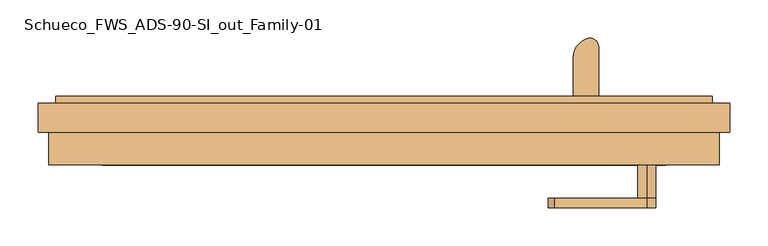
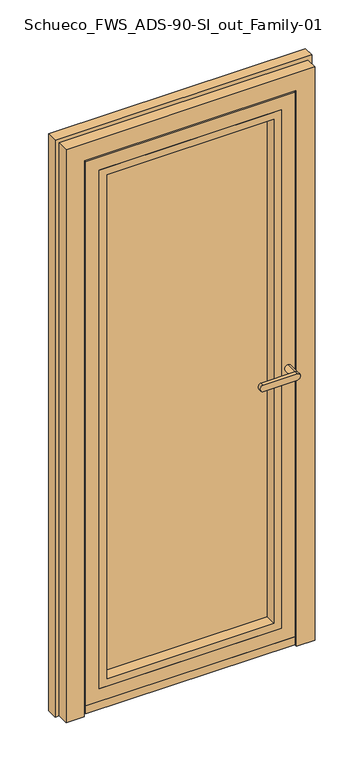
"""IFC4 building model written with IfcOpenShell, lengths in millimetres: door geometry, Schueco_FWS_ADS-90-SI_out_Family-01 : FWS SI insert unit."""

from ifc_helpers import new_model, si_unit, point, frame, frame_2d, origin, place, context, project, spatial, polyline, circle_curve, ellipse_curve, trimmed, segment, composite_curve, outline, extrude, faceted_brep, source, transform, mapped, element, save
from ifc_brep_helpers import plane_surface, cylinder_surface, extruded_surface, advanced_brep


def schueco_fws_ads_90_si_out_family_01_926161e4(model_context):
    return source(origin(), model_context, "Body", "SolidModel", [
        extrude(outline(composite_curve([segment(polyline([(248.3326764, 8.9997177), (248.3326764, 59.1618682)]), True, "CONTINUOUS"), segment(trimmed(circle_curve(frame_2d((275.5110941, 59.1618682)), 27.1784177), [point((248.3326764, 59.1618682))], [point((265.9739985, 84.6120194))], False, "CARTESIAN"), True, "CONTINUOUS"), segment(trimmed(circle_curve(frame_2d((270.0514995, 73.7310321)), 11.6198924), [point((265.9739985, 84.6120194))], [point((281.6713919, 73.7310321))], False, "CARTESIAN"), True, "CONTINUOUS"), segment(polyline([(281.6713919, 73.7310321), (281.6713919, 8.9997177), (248.3326764, 8.9997177)]), True, "CONTINUOUS")], self_intersect=False)), frame((0.0, 0.0, 2043.9340013), z_axis=(0.0, 0.0, 1.0), x_axis=(1.0, 0.0, 0.0)), (0.0, 0.0, 1.0), 4.0),
        extrude(outline(polyline([(248.3326764, 12.9997177), (281.6713919, 12.9997177), (281.6713919, 8.9997177), (248.3326764, 8.9997177), (248.3326764, 12.9997177)])), frame((0.0, 0.0, 2013.9340013), z_axis=(0.0, 0.0, 1.0), x_axis=(1.0, 0.0, 0.0)), (0.0, 0.0, 1.0), 30.0),
        extrude(outline(polyline([(248.3326764, 12.9997177), (281.6713919, 12.9997177), (281.6713919, 8.9997177), (248.3326764, 8.9997177), (248.3326764, 12.9997177)])), frame((0.0, 0.0, 56.9340013), z_axis=(0.0, 0.0, 1.0), x_axis=(1.0, 0.0, 0.0)), (0.0, 0.0, 1.0), 30.0),
        extrude(outline(composite_curve([segment(polyline([(248.3326764, 8.9997177), (248.3326764, 59.1618682)]), True, "CONTINUOUS"), segment(trimmed(circle_curve(frame_2d((275.5110941, 59.1618682)), 27.1784177), [point((248.3326764, 59.1618682))], [point((265.9739985, 84.6120194))], False, "CARTESIAN"), True, "CONTINUOUS"), segment(trimmed(circle_curve(frame_2d((270.0514995, 73.7310321)), 11.6198924), [point((265.9739985, 84.6120194))], [point((281.6713919, 73.7310321))], False, "CARTESIAN"), True, "CONTINUOUS"), segment(polyline([(281.6713919, 73.7310321), (281.6713919, 8.9997177), (248.3326764, 8.9997177)]), True, "CONTINUOUS")], self_intersect=False)), frame((0.0, 0.0, 52.9340013), z_axis=(0.0, 0.0, 1.0), x_axis=(1.0, 0.0, 0.0)), (0.0, 0.0, 1.0), 4.0),
        advanced_brep(
        [(277.717076, 57.5977179, 2043.9340013), (252.282924, 72.2821425, 2043.9340013), (277.717076, 57.5977179, 56.9340013), (252.282924, 72.2821425, 56.9340013)],
        [
            (0, 1, ellipse_curve(frame((265.0, 64.9399302, 2043.9340013), z_axis=(0.0, 0.0, 1.0000000000000002), x_axis=(0.5000002582658958, 0.866025254674503, 0.0)), 21.5840887, 14.6844171)),
            (1, 0, ellipse_curve(frame((265.0, 64.9399302, 2043.9340013), z_axis=(0.0, 0.0, 1.0000000000000002), x_axis=(0.5000002582658958, 0.866025254674503, 0.0)), 21.5840887, 14.6844171)),
            (2, 3, ellipse_curve(frame((265.0, 64.9399302, 56.9340013), z_axis=(0.0, 0.0, -1.0000000000000002), x_axis=(-0.866025254674503, 0.5000002582658958, 0.0)), 14.6844171, 21.5840887)),
            (3, 2, ellipse_curve(frame((265.0, 64.9399302, 56.9340013), z_axis=(0.0, 0.0, -1.0000000000000002), x_axis=(-0.866025254674503, 0.5000002582658958, 0.0)), 14.6844171, 21.5840887)),
            (0, 2),
            (3, 1),
        ],
        [
            plane_surface(frame((252.282924, 72.2821425, 2043.9340013), z_axis=(0.0, 0.0, 1.0000000000000002), x_axis=(0.5000002582658958, 0.866025254674503, 0.0))),
            plane_surface(frame((252.282924, 72.2821425, 56.9340013), z_axis=(0.0, 0.0, -1.0000000000000002), x_axis=(-0.5000002582658958, -0.866025254674503, 0.0))),
            extruded_surface(trimmed(ellipse_curve(frame((265.0, 64.9399302, 56.9340013), z_axis=(0.0, 0.0, -1.0000000000000002), x_axis=(-0.866025254674503, 0.5000002582658958, 0.0)), 14.6844171, 21.5840887), [point((252.282924, 72.2821425, 56.9340013))], [point((277.717076, 57.5977179, 56.9340013))], True, "CARTESIAN"), (0.0, 0.0, -1987.0), 1987.0),
            extruded_surface(trimmed(ellipse_curve(frame((265.0, 64.9399302, 56.9340013), z_axis=(0.0, 0.0, -1.0000000000000002), x_axis=(-0.866025254674503, 0.5000002582658958, 0.0)), 14.6844171, 21.5840887), [point((277.717076, 57.5977179, 56.9340013))], [point((252.282924, 72.2821425, 56.9340013))], True, "CARTESIAN"), (0.0, 0.0, -1987.0), 1987.0),
        ],
        [
            (0, [[1, 2]]),
            (1, [[3, 4]]),
            (2, [[5, -4, 6, -1]]),
            (3, [[-6, -3, -5, -2]]),
        ],
    ),
        advanced_brep(
        [(345.0, -137.0002518, 1038.0113692), (345.0, -137.0002518, 1061.9886308), (223.3382074, -137.0002518, 1061.9886308), (223.3382074, -137.0002518, 1038.0113692), (345.0, -124.5001648, 1061.9886308), (345.0, -124.5001648, 1038.0113692), (223.3382074, -124.5001648, 1038.0113692), (223.3382074, -124.5001648, 1061.9886308), (345.0, -81.0002823, 1038.0113692), (345.0, -81.0002823, 1061.9886308)],
        [
            (0, 1, circle_curve(frame((345.0, -137.0002518, 1050.0), z_axis=(0.0, -1.0, 0.0), x_axis=(0.0, 0.0, 1.0)), 11.9886308)),
            (1, 2),
            (2, 3, ellipse_curve(frame((223.3382074, -137.0002518, 1050.0), z_axis=(0.0, -1.0, 0.0), x_axis=(0.0, 0.0, -1.0)), 11.9886308, 7.9050795)),
            (3, 0),
            (4, 5, circle_curve(frame((345.0, -124.5001648, 1050.0), z_axis=(0.0, -1.0, 0.0), x_axis=(0.0, 0.0, 1.0)), 11.9886308)),
            (5, 6),
            (6, 7, ellipse_curve(frame((223.3382074, -124.5001648, 1050.0), z_axis=(0.0, 1.0, 0.0), x_axis=(0.0, 0.0, -1.0)), 11.9886308, 7.9050795)),
            (7, 4),
            (3, 6),
            (5, 0),
            (2, 7),
            (1, 4),
            (5, 4, circle_curve(frame((345.0, -124.5001648, 1050.0), z_axis=(0.0, -1.0, 0.0), x_axis=(0.0, 0.0, 1.0)), 11.9886308)),
            (8, 9, circle_curve(frame((345.0, -81.0002823, 1050.0), z_axis=(0.0, 1.0, 0.0), x_axis=(0.0, 0.0, 1.0)), 11.9886308)),
            (9, 8, circle_curve(frame((345.0, -81.0002823, 1050.0), z_axis=(0.0, 1.0, 0.0), x_axis=(0.0, 0.0, 1.0)), 11.9886308)),
            (8, 5),
            (4, 9),
        ],
        [
            plane_surface(frame((223.3382074, -137.0002518, 1038.0113692), z_axis=(0.0, -1.0, 0.0), x_axis=(-1.0, 0.0, 0.0))),
            plane_surface(frame((223.3382074, -124.5001648, 1038.0113692), z_axis=(0.0, 1.0, 0.0), x_axis=(1.0, 0.0, 0.0))),
            plane_surface(frame((345.0, -137.0002518, 1038.0113692), z_axis=(0.0, 0.0, -1.0), x_axis=(0.0, 1.0, 0.0))),
            extruded_surface(trimmed(ellipse_curve(frame((223.3382074, -124.5001648, 1050.0), z_axis=(0.0, 1.0, 0.0), x_axis=(0.0, 0.0, -1.0)), 11.9886308, 7.9050795), [point((223.3382074, -124.5001648, 1038.0113692))], [point((223.3382074, -124.5001648, 1061.9886308))], True, "CARTESIAN"), (0.0, 12.500086999999994, 0.0), 12.500086999999994),
            plane_surface(frame((223.3382074, -137.0002518, 1061.9886308), z_axis=(0.0, 0.0, 1.0), x_axis=(0.0, 1.0, 0.0))),
            cylinder_surface(frame((345.0, -124.5001648, 1050.0), z_axis=(0.0, -1.0, 0.0), x_axis=(0.0, 0.0, 1.0)), 11.9886308),
            plane_surface(frame((345.0, -81.0002823, 1061.9886308), z_axis=(0.0, 1.0, 0.0), x_axis=(-1.0, 0.0, 0.0))),
            cylinder_surface(frame((345.0, -81.0002823, 1050.0), z_axis=(0.0, -1.0, 0.0), x_axis=(0.0, 0.0, 1.0)), 11.9886308),
        ],
        [
            (0, [[1, 2, 3, 4]]),
            (1, [[5, 6, 7, 8]]),
            (2, [[9, -6, 10, -4]]),
            (3, [[11, -7, -9, -3]]),
            (4, [[12, -8, -11, -2]]),
            (5, [[-10, 13, -12, -1]]),
            (6, [[14, 15]]),
            (7, [[16, -5, 17, -14]]),
            (7, [[-17, -13, -16, -15]]),
        ],
    ),
        extrude(outline(polyline([(86.0, 322.0), (2022.0, 322.0), (2022.0, -322.0), (86.0, -322.0), (86.0, 322.0)]), holes=[polyline([(113.0, -295.0), (1995.0, -295.0), (1995.0, 295.0), (113.0, 295.0), (113.0, -295.0)])]), frame((0.0, -81.0002823, 0.0), z_axis=(0.0, 1.0, 0.0), x_axis=(0.0, 0.0, 1.0)), (0.0, 0.0, 1.0), 41.0000097),
        faceted_brep([(-370.0, -81.0002823, 2070.0), (-370.0, -72.5000065, 2070.0), (-370.0, -72.5000065, 38.0), (-370.0, -81.0002823, 38.0), (370.0, -72.5000065, 38.0), (370.0, -81.0002823, 38.0), (382.0, -72.5000065, 26.0), (382.0, -72.5000065, 2082.0), (-382.0, -72.5000065, 2082.0), (-382.0, -72.5000065, 26.0), (370.0, -72.5000065, 2070.0), (370.0, -81.0002823, 2070.0), (-322.0, -81.0002823, 86.0), (-322.0, -81.0002823, 2022.0), (322.0, -81.0002823, 2022.0), (322.0, -81.0002823, 86.0), (-322.0, -2.0002726, 2022.0), (-322.0, -2.0002726, 86.0), (322.0, -2.0002726, 86.0), (322.0, -2.0002726, 2022.0), (-297.0, -2.0002726, 111.0), (-297.0, -2.0002726, 1997.0), (297.0, -2.0002726, 1997.0), (297.0, -2.0002726, 111.0), (-297.0, 8.9997177, 1997.0), (-297.0, 8.9997177, 111.0), (297.0, 8.9997177, 111.0), (297.0, 8.9997177, 1997.0), (-400.0, 8.9997177, 8.0), (-400.0, 8.9997177, 2100.0), (400.0, 8.9997177, 2100.0), (400.0, 8.9997177, 8.0), (-400.0, 0.4997603, 2100.0), (-400.0, 0.4997603, 8.0), (400.0, 0.4997603, 8.0), (400.0, 0.4997603, 2100.0), (-382.0, 0.4997603, 26.0), (-382.0, 0.4997603, 2082.0), (382.0, 0.4997603, 2082.0), (382.0, 0.4997603, 26.0)], [[[0, 1, 2, 3]], [[3, 2, 4, 5]], [[6, 7, 8, 9], [2, 1, 10, 4]], [[5, 4, 10, 11]], [[5, 11, 0, 3], [12, 13, 14, 15]], [[16, 13, 12, 17]], [[17, 12, 15, 18]], [[18, 15, 14, 19]], [[18, 19, 16, 17], [20, 21, 22, 23]], [[24, 21, 20, 25]], [[25, 20, 23, 26]], [[26, 23, 22, 27]], [[28, 29, 30, 31], [26, 27, 24, 25]], [[32, 29, 28, 33]], [[33, 28, 31, 34]], [[34, 31, 30, 35]], [[34, 35, 32, 33], [36, 37, 38, 39]], [[8, 37, 36, 9]], [[9, 36, 39, 6]], [[6, 39, 38, 7]], [[11, 10, 1, 0]], [[19, 14, 13, 16]], [[27, 22, 21, 24]], [[35, 30, 29, 32]], [[7, 38, 37, 8]]]),
        extrude(outline(polyline([(322.0, -40.0002726), (-322.0, -40.0002726), (-322.0, -2.0002726), (322.0, -2.0002726), (322.0, -40.0002726)])), frame((0.0, 0.0, 86.0), z_axis=(0.0, 0.0, 1.0), x_axis=(1.0, 0.0, 0.0)), (0.0, 0.0, 1.0), 1936.0),
        extrude(outline(composite_curve([segment(polyline([(-37.1566288, 3.0385292), (-37.1566288, 26.0), (-15.8518963, 26.0), (-15.8518963, 3.0385292)]), True, "CONTINUOUS"), segment(trimmed(circle_curve(frame_2d((-26.5042625, 20.1647327)), 20.1687817), [point((-15.8518963, 3.0385292))], [point((-37.1566288, 3.0385292))], False, "CARTESIAN"), True, "CONTINUOUS")], self_intersect=False)), frame((-370.0, 0.0, 0.0), z_axis=(1.0, 0.0, 0.0), x_axis=(0.0, 1.0, 0.0)), (0.0, 0.0, 1.0), 740.0),
        extrude(outline(polyline([(-370.0, -81.0002823), (-370.0, -72.5003249), (370.0, -72.5003249), (370.0, -81.0002823), (-370.0, -81.0002823)])), frame((0.0, 0.0, 8.0), z_axis=(0.0, 0.0, 1.0), x_axis=(1.0, 0.0, 0.0)), (0.0, 0.0, 1.0), 30.0),
        faceted_brep([(430.999943, 8.9997177, 2130.999943), (430.999943, 0.0, 2130.999943), (430.999943, 0.0, 0.0), (430.999943, 8.9997177, 0.0), (-454.0, 0.0, 0.0), (-454.0, 0.0, 2154.0), (454.0, 0.0, 2154.0), (454.0, 0.0, 0.0), (-430.999943, 0.0, 2130.999943), (-430.999943, 0.0, 0.0), (454.0, -38.0, 0.0), (440.0, -38.0, 0.0), (440.0, -81.0002823, 0.0), (375.0001013, -81.0002823, 0.0), (375.0001013, -72.5000065, 0.0), (393.0000155, -72.5000065, 0.0), (393.0000155, 0.4997603, 0.0), (405.0000266, 0.4997603, 0.0), (405.0000266, 8.9997177, 0.0), (-405.0000266, 8.9997177, 0.0), (-430.999943, 8.9997177, 0.0), (-430.999943, 8.9997177, 2130.999943), (405.0000266, 8.9997177, 2105.0000266), (-405.0000266, 8.9997177, 2105.0000266), (375.0001013, -81.0002823, 2075.0001013), (375.0001013, -72.5000065, 2075.0001013), (-375.0001013, -72.5000065, 0.0), (-393.0000155, -72.5000065, 0.0), (-393.0000155, -72.5000065, 2093.0000155), (393.0000155, -72.5000065, 2093.0000155), (-375.0001013, -72.5000065, 2075.0001013), (-440.0, -81.0002823, 0.0), (-375.0001013, -81.0002823, 0.0), (-375.0001013, -81.0002823, 2075.0001013), (440.0, -81.0002823, 2140.0), (-440.0, -81.0002823, 2140.0), (440.0, -38.0, 2140.0), (-454.0, -38.0, 0.0), (-440.0, -38.0, 0.0), (-440.0, -38.0, 2140.0), (454.0, -38.0, 2154.0), (-454.0, -38.0, 2154.0), (-405.0000266, 0.4997603, 0.0), (-393.0000155, 0.4997603, 0.0), (405.0000266, 0.4997603, 2105.0000266), (-405.0000266, 0.4997603, 2105.0000266), (393.0000155, 0.4997603, 2093.0000155), (-393.0000155, 0.4997603, 2093.0000155)], [[[0, 1, 2, 3]], [[4, 5, 6, 7, 2, 1, 8, 9]], [[3, 2, 7, 10, 11, 12, 13, 14, 15, 16, 17, 18]], [[19, 20, 21, 0, 3, 18, 22, 23]], [[24, 25, 14, 13]], [[26, 27, 28, 29, 15, 14, 25, 30]], [[31, 32, 33, 24, 13, 12, 34, 35]], [[34, 12, 11, 36]], [[37, 38, 39, 36, 11, 10, 40, 41]], [[4, 9, 20, 19, 42, 43, 27, 26, 32, 31, 38, 37]], [[20, 9, 8, 21]], [[18, 17, 44, 22]], [[42, 19, 23, 45]], [[32, 26, 30, 33]], [[31, 35, 39, 38]], [[4, 37, 41, 5]], [[6, 40, 10, 7]], [[43, 42, 45, 44, 17, 16, 46, 47]], [[16, 15, 29, 46]], [[27, 43, 47, 28]], [[21, 8, 1, 0]], [[33, 30, 25, 24]], [[35, 34, 36, 39]], [[23, 22, 44, 45]], [[5, 41, 40, 6]], [[47, 46, 29, 28]]]),
    ])


if __name__ == "__main__":
    model = new_model("IFC4")
    model_context = context("Model", 3, world=origin())
    ifc_project = project(units=[si_unit("LENGTHUNIT", "METRE", prefix="MILLI")], contexts=[model_context])
    site = spatial("IfcSite", under=ifc_project)
    building = spatial("IfcBuilding", under=site)
    placement = place(None, origin())
    schueco_fws_ads_90_si_out_family_01_shape = schueco_fws_ads_90_si_out_family_01_926161e4(model_context)
    element("IfcDoor", 1, ObjectType="Schueco_FWS_ADS-90-SI_out_Family-01 : FWS SI insert unit", at=placement, inside=building, context=model_context, shape_type="MappedRepresentation", body=[
        mapped(schueco_fws_ads_90_si_out_family_01_shape, transform((0.0, 0.0, 0.0), x_axis=(1.0, 0.0, 0.0), y_axis=(0.0, 1.0, 0.0), z_axis=(0.0, 0.0, 1.0))),
    ])
    save(model, "model.ifc")

# Revit data of these elements
# Type "Schueco_FWS_ADS-90-SI_out_Family-01 : FWS SI insert unit"
#   Type Mark = "38"
#   __NOTE__ = "Data describes the optimum values of the entire system. The properites of a selected design option have to be determined on an individual basis!"
#   Wind load resistance = "Class C3"
#   Watertightness = "Class 7A"
#   Thermal insulation = "Uf = 1.2 W/(m²K)"
#   Sound insulation = "..."
#   Schueco thermal insulation standard = "Highly thermally insulated"
#   Opening type = "Outward-opening, Flush-fitted"
#   Model = "Schueco ADS 90.SI"
#   Mechanical loading = "Class 3"
#   Maximum leaf width in mm = "1600"
#   Maximum leaf weight in kg = "160"
#   Maximum leaf height in mm = "2500"
#   Material = "Aluminium"
#   Construction Type = "Door, single-leaf, outward-opening"
#   Manufacturer = "Schueco International KG"
#   Long term functionality = "..."
#   Glazing data = "Triple glazing 38mm"
#   Façade insert unit = "yes"
#   Family creation date = "08.2017"
#   Description = "Schueco Aluminium Door System (ADS)"
#   Burglar resistance = "Class RC 3"
#   Areas of use = "Public buildings, Side entrance"
#   Analytic Construction = "<None>"
#   Air permeability = "Class 4"
#   Width [instance default] = 612.144 mm
#   Leaf opening angle [instance default] = 0.00°
#   IOf_T = 38 mm
#   Height [instance default] = 2012.289 mm
#   Glazing area [instance default] = 0.520049 m²
#   Distance from bottom to handles [instance default] = 1050 mm
#   Clear opening width [instance default] = 454.144 mm
#   Standard threshold = no
#   Low level threshold = yes
#   Handles = yes
#   Glass = none
#   Frame = Alu
#   Fittings = none
# Element 1 (IfcDoor, "Schueco_FWS_ADS-90-SI_out_Family-01 : FWS SI insert unit")
#   Width = 908 mm
#   Height = 2154 mm
#   Glazing area = 1.12028 m²
#   Clear opening width = 750 mm
#   Materials on its faces: "Alu", "Glass"
# Materials
#   "Alu": class "Glas", colour RGB 140 140 140, transparency 0
#   "Glass": class "Glass", colour RGB 128 128 255, transparency 0.75, Description = "Soda Lime Glass", Cost = 0
